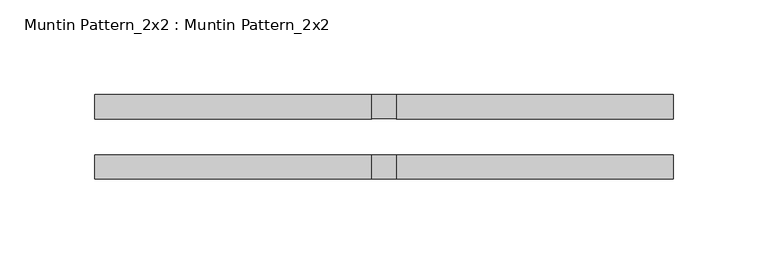
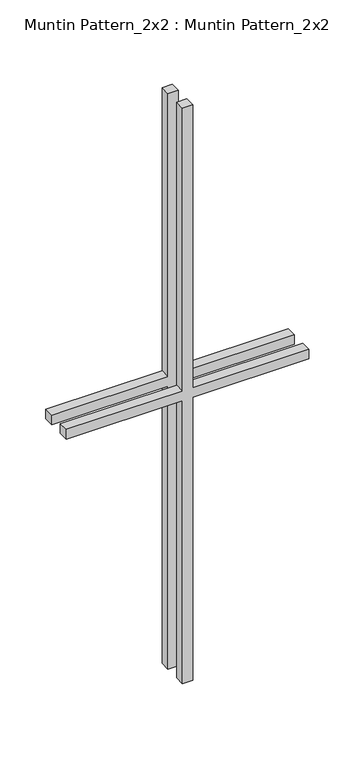
"""IFC4 building model written with IfcOpenShell, lengths in millimetres: proxy geometry, Muntin Pattern_2x2 : Muntin Pattern_2x2."""

import ifcopenshell
import ifcopenshell.guid

model = None  # the IFC model being written
_history = None  # IfcOwnerHistory: only IFC2X3 demands one
_inside = {}  # id of a spatial element -> (the spatial element, [elements in it])
_under = {}  # id of a project, library or spatial element -> (it, [spatial elements below it])
_declared = {}  # id of a project -> (the project, [libraries it declares])
_typed = {}  # id of a type object -> (the type object, [elements of that type])
_made_of = {}  # id of a material, layer set ... -> (it, [elements and type objects made of it])


def new_model(schema):
    """Start an empty IFC model of exactly this schema.

    Asked for "IFC4X3", IfcOpenShell would pick the latest addendum, in which some entities
    have other attributes; the version numbers below select the first issue.
    IFC2X3 requires an IfcOwnerHistory on every rooted entity: one is made here for all.
    """
    global model, _history
    if schema == "IFC4X3":
        model = ifcopenshell.file(schema_version=(4, 3, 0, 0))
    else:
        model = ifcopenshell.file(schema=schema)
    _inside.clear()
    _under.clear()
    _declared.clear()
    _typed.clear()
    _made_of.clear()
    _history = None
    if model.schema == "IFC2X3":
        org = make("IfcOrganization", Name="unknown")
        user = make(
            "IfcPersonAndOrganization",
            ThePerson=make("IfcPerson", FamilyName="unknown"),
            TheOrganization=org,
        )
        app = make(
            "IfcApplication",
            ApplicationDeveloper=org,
            Version="unknown",
            ApplicationFullName="unknown",
            ApplicationIdentifier="unknown",
        )
        _history = make(
            "IfcOwnerHistory",
            OwningUser=user,
            OwningApplication=app,
            ChangeAction="ADDED",
            CreationDate=0,
        )
    return model


def make(cls, **values):
    """One entity of the class cls with the attributes given. An attribute that is None is left unset."""
    return model.create_entity(
        cls, **{name: value for name, value in values.items() if value is not None}
    )


def rooted(cls, **values):
    """An entity with a GlobalId (a new one), such as an element, a storey or a relation."""
    return make(cls, GlobalId=ifcopenshell.guid.new(), OwnerHistory=_history, **values)


def si_unit(unit_type, name, prefix=None):
    """IfcSIUnit, for example si_unit("LENGTHUNIT", "METRE", prefix="MILLI")."""
    return make("IfcSIUnit", UnitType=unit_type, Prefix=prefix, Name=name)


def assignment(units):
    """IfcUnitAssignment: the units of a project."""
    return None if units is None else make("IfcUnitAssignment", Units=units)


def point(xyz):
    """IfcCartesianPoint."""
    return None if xyz is None else make("IfcCartesianPoint", Coordinates=xyz)


def direction(xyz):
    """IfcDirection."""
    return None if xyz is None else make("IfcDirection", DirectionRatios=xyz)


def frame(location, z_axis=None, x_axis=None):
    """IfcAxis2Placement3D, a coordinate frame: its origin and axes. An axis left out is left unset."""
    return make(
        "IfcAxis2Placement3D",
        Location=point(location),
        Axis=direction(z_axis),
        RefDirection=direction(x_axis),
    )


def origin():
    """The frame at (0, 0, 0) with its axes left unset."""
    return frame((0.0, 0.0, 0.0))


def place(relative_to, where):
    """IfcLocalPlacement: puts the frame where relative to a parent placement (None: the world)."""
    return make(
        "IfcLocalPlacement", PlacementRelTo=relative_to, RelativePlacement=where
    )


def context(
    kind, dimensions, precision=None, world=None, true_north=None, identifier=None
):
    """IfcGeometricRepresentationContext, for example the 3D "Model" context."""
    return make(
        "IfcGeometricRepresentationContext",
        ContextIdentifier=identifier,
        ContextType=kind,
        CoordinateSpaceDimension=dimensions,
        Precision=precision,
        WorldCoordinateSystem=world,
        TrueNorth=true_north,
    )


def project(units=None, contexts=None):
    """IfcProject with its units and contexts."""
    return rooted(
        "IfcProject",
        Name="project",
        RepresentationContexts=contexts,
        UnitsInContext=assignment(units),
    )


def spatial(cls, under=None, at=None, **own):
    """A site, building, storey or space (cls), placed at a placement, below another one or the project."""
    s = rooted(cls, ObjectPlacement=at, **own)
    if under is not None:
        _under.setdefault(under.id(), (under, []))[1].append(s)
    return s


def polyline(points):
    """IfcPolyline through the points."""
    return make("IfcPolyline", Points=[point(p) for p in points])


def outline(outer, holes=None, kind="AREA"):
    """IfcArbitraryClosedProfileDef: a profile drawn as a closed curve; with holes, ...WithVoids."""
    if holes is None:
        return make("IfcArbitraryClosedProfileDef", ProfileType=kind, OuterCurve=outer)
    return make(
        "IfcArbitraryProfileDefWithVoids",
        ProfileType=kind,
        OuterCurve=outer,
        InnerCurves=holes,
    )


def extrude(swept, where, along, depth):
    """IfcExtrudedAreaSolid: the profile swept, set in the frame where, extruded along a direction by depth."""
    return make(
        "IfcExtrudedAreaSolid",
        SweptArea=swept,
        Position=where,
        ExtrudedDirection=direction(along),
        Depth=depth,
    )


def shape(context_of_items, identifier, shape_type, items):
    """IfcShapeRepresentation: the items that make up one representation, for example the "Body"."""
    return make(
        "IfcShapeRepresentation",
        ContextOfItems=context_of_items,
        RepresentationIdentifier=identifier,
        RepresentationType=shape_type,
        Items=items,
    )


def source(mapping_origin, context_of_items, identifier, shape_type, items):
    """IfcRepresentationMap: a shape defined once, which mapped items show again and again."""
    return make(
        "IfcRepresentationMap",
        MappingOrigin=mapping_origin,
        MappedRepresentation=shape(context_of_items, identifier, shape_type, items),
    )


def transform(
    local_origin,
    x_axis=None,
    y_axis=None,
    z_axis=None,
    scale=None,
    scale2=None,
    scale3=None,
    uniform=True,
):
    """IfcCartesianTransformationOperator3D, or its non-uniform kind. x_axis, y_axis, z_axis: its Axis1, 2, 3."""
    if uniform:
        return make(
            "IfcCartesianTransformationOperator3D",
            Axis1=direction(x_axis),
            Axis2=direction(y_axis),
            LocalOrigin=point(local_origin),
            Scale=scale,
            Axis3=direction(z_axis),
        )
    return make(
        "IfcCartesianTransformationOperator3DnonUniform",
        Axis1=direction(x_axis),
        Axis2=direction(y_axis),
        LocalOrigin=point(local_origin),
        Scale=scale,
        Axis3=direction(z_axis),
        Scale2=scale2,
        Scale3=scale3,
    )


def mapped(mapping_source, mapping_target):
    """IfcMappedItem: shows the shape of a source again, moved by a transform."""
    return make(
        "IfcMappedItem", MappingSource=mapping_source, MappingTarget=mapping_target
    )


def made_of(thing, what):
    """Note that an element or type object is made of a material, layer set ...; save() writes the relation."""
    if what is not None:
        _made_of.setdefault(what.id(), (what, []))[1].append(thing)
    return thing


def element(
    cls,
    number,
    at=None,
    inside=None,
    cuts=None,
    type_object=None,
    material=None,
    context=None,
    identifier="Body",
    shape_type=None,
    held_by="IfcProductDefinitionShape",
    body=None,
    shapes=None,
    **own,
):
    """One element of the class cls, such as IfcWall. Its Tag is "e" and its number.

    at: its placement. inside: the storey or other place that contains it. cuts: it is an
    opening in that element (IfcRelVoidsElement). A single representation is given by context,
    identifier, shape_type and body (its items); several are given by shapes. held_by: the class
    of the entity that holds the representations. save() writes the other relations.
    """
    e = rooted(cls, Tag="e%d" % number, ObjectPlacement=at, **own)
    if body is not None:
        shapes = [shape(context, identifier, shape_type, body)]
    if shapes is not None:
        e.Representation = make(held_by, Representations=shapes)
    if inside is not None:
        _inside.setdefault(inside.id(), (inside, []))[1].append(e)
    if cuts is not None:
        rooted(
            "IfcRelVoidsElement", RelatingBuildingElement=cuts, RelatedOpeningElement=e
        )
    if type_object is not None:
        _typed.setdefault(type_object.id(), (type_object, []))[1].append(e)
    return made_of(e, material)


def aggregate(whole, parts):
    """IfcRelAggregates: a whole, such as a stair, and the parts it consists of."""
    return rooted("IfcRelAggregates", RelatingObject=whole, RelatedObjects=parts)


def save(model, path):
    """Write the relations noted so far, then the file.

    IfcRelAggregates (storeys below a building ...), IfcRelContainedInSpatialStructure (elements
    in a storey), IfcRelDefinesByType, IfcRelAssociatesMaterial and IfcRelDeclares: one each for
    every whole, place, type object, material and project.
    """
    for whole, parts in _under.values():
        aggregate(whole, parts)
    for where, things in _inside.values():
        rooted(
            "IfcRelContainedInSpatialStructure",
            RelatedElements=things,
            RelatingStructure=where,
        )
    for kind, things in _typed.values():
        rooted("IfcRelDefinesByType", RelatedObjects=things, RelatingType=kind)
    for what, things in _made_of.values():
        rooted("IfcRelAssociatesMaterial", RelatedObjects=things, RelatingMaterial=what)
    for by, libraries in _declared.values():
        rooted("IfcRelDeclares", RelatingContext=by, RelatedDefinitions=libraries)
    model.write(path)


def muntin_pattern_2x2_muntin_pattern_2x2_e055f423(model_context):
    return source(origin(), model_context, "Body", "SweptSolid", [
        extrude(outline(polyline([(388.9375, -6.35), (388.9375, -152.4), (376.2375, -152.4), (376.2375, -6.35), (0.0, -6.35), (0.0, 6.35), (376.2375, 6.35), (376.2375, 152.4), (388.9375, 152.4), (388.9375, 6.35), (765.175, 6.35), (765.175, -6.35), (388.9375, -6.35)])), frame((0.0, 9.525, 0.0), z_axis=(0.0, 1.0, 0.0), x_axis=(0.0, 0.0, 1.0)), (0.0, 0.0, 1.0), 12.7),
        extrude(outline(polyline([(388.9375, -6.35), (388.9375, -152.4), (376.2375, -152.4), (376.2375, -6.35), (0.0, -6.35), (0.0, 6.35), (376.2375, 6.35), (376.2375, 152.4), (388.9375, 152.4), (388.9375, 6.35), (765.175, 6.35), (765.175, -6.35), (388.9375, -6.35)])), frame((0.0, -22.225, 0.0), z_axis=(0.0, 1.0, 0.0), x_axis=(0.0, 0.0, 1.0)), (0.0, 0.0, 1.0), 12.7),
    ])


if __name__ == "__main__":
    model = new_model("IFC4")
    model_context = context("Model", 3, world=origin())
    ifc_project = project(units=[si_unit("LENGTHUNIT", "METRE", prefix="MILLI")], contexts=[model_context])
    site = spatial("IfcSite", under=ifc_project)
    building = spatial("IfcBuilding", under=site)
    placement = place(None, origin())
    muntin_pattern_2x2_muntin_pattern_2x2_shape = muntin_pattern_2x2_muntin_pattern_2x2_e055f423(model_context)
    element("IfcBuildingElementProxy", 1, Name="Muntin Pattern_2x2 : Muntin Pattern_2x2", ObjectType="Muntin Pattern_2x2 : Muntin Pattern_2x2", at=placement, inside=building, context=model_context, shape_type="MappedRepresentation", body=[
        mapped(muntin_pattern_2x2_muntin_pattern_2x2_shape, transform((0.0, 0.0, 0.0), x_axis=(1.0, 0.0, 0.0), y_axis=(0.0, 1.0, 0.0), z_axis=(0.0, 0.0, 1.0))),
    ])
    save(model, "model.ifc")

# Revit data of these elements
# Type "Muntin Pattern_2x2 : Muntin Pattern_2x2"
#   Width [instance default] = 4' - 0"
#   Thickness = 0' - 0 1/2"
#   Height [instance default] = 4' - 0"
#   Distance = 0' - 0 3/4"
#   Interior Material [instance default] = none
#   Exterior Material [instance default] = none
# Element 1 (IfcBuildingElementProxy, "Muntin Pattern_2x2 : Muntin Pattern_2x2")
#   Width = 1' - 0"
#   Height = 2' - 6 1/8"
#   Interior Material = 1X WOOD COMPOSITE TRIM
#   Exterior Material = 1X WOOD COMPOSITE TRIM
#   Materials on its faces: "1X WOOD COMPOSITE TRIM"
# Materials
#   "1X WOOD COMPOSITE TRIM": class "Generic", colour RGB 88 61 61, transparency 0, Cost = 0
